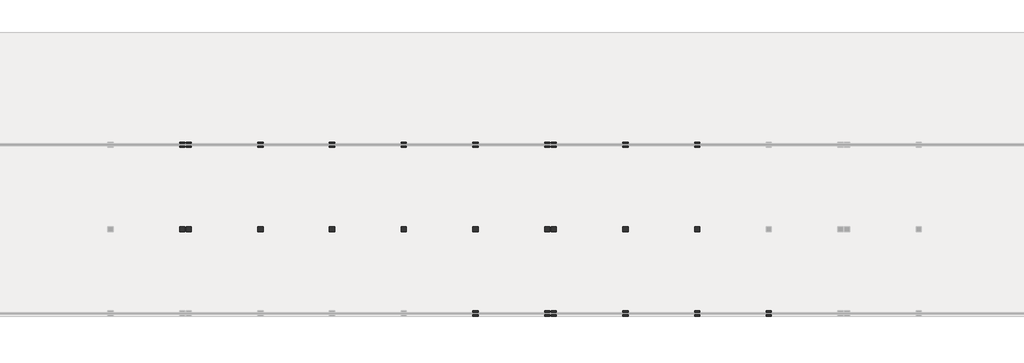
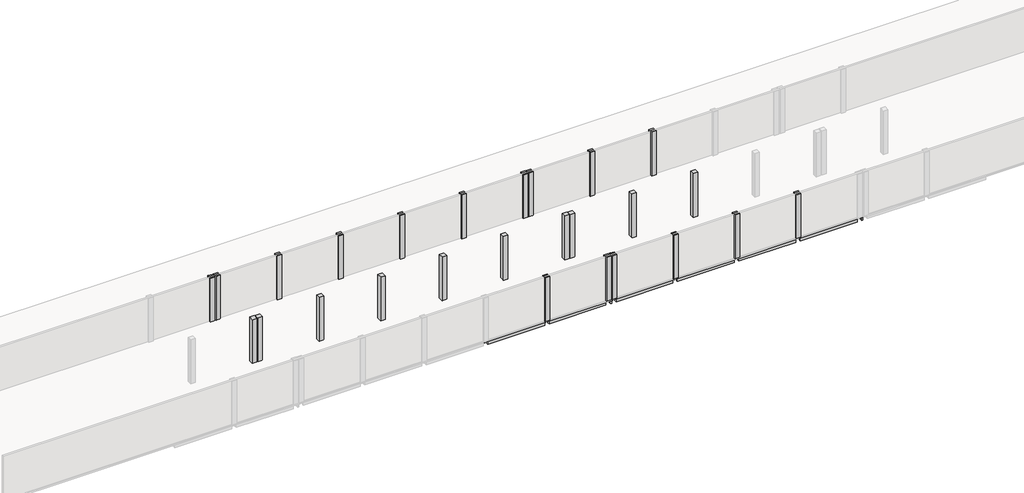
# One storey, part 2 of 4: 52 beams, 26 columns.
"""IFC4 building model written with IfcOpenShell, lengths in millimetres."""

from ifc_helpers import new_model, si_unit, frame, origin, place, context, project, spatial, polyline, outline, extrude, element, save

model = new_model("IFC4")

# Units and contexts
model_context = context("Model", 3, world=origin())
ifc_project = project(units=[si_unit("LENGTHUNIT", "METRE", prefix="MILLI")], contexts=[model_context])

# Site, building, storey
site = spatial("IfcSite", under=ifc_project)
building = spatial("IfcBuilding", under=site)
storey = spatial("IfcBuildingStorey", under=building, Name="03_T.O.C_1", Elevation=6949.9618634)

# Beams
placement = place(None, origin())
element("IfcBeam", 1, ObjectType="RC Beam_Rectangular : H_SB_AR_S16_B300xH600", at=placement, inside=storey, context=model_context, shape_type="SweptSolid", body=[
    extrude(outline(polyline([(35030.0, -6150.4791411), (35030.0, -5850.4791411), (35180.0, -5850.4791411), (35180.0, -6150.4791411), (35030.0, -6150.4791411)])), frame((0.0, 0.0, 6349.9618634), z_axis=(0.0, 0.0, 1.0), x_axis=(1.0, 0.0, 0.0)), (0.0, 0.0, 1.0), 499.0),
])
element("IfcBeam", 2, ObjectType="RC Beam_Rectangular : H_SB_AR_S16_B300xH600", at=placement, inside=storey, context=model_context, shape_type="SweptSolid", body=[
    extrude(outline(polyline([(35780.0, -6150.4791411), (35780.0, -5850.4791411), (43380.0, -5850.4791411), (43380.0, -6150.4791411), (35780.0, -6150.4791411)])), frame((0.0, 0.0, 6349.9618634), z_axis=(0.0, 0.0, 1.0), x_axis=(1.0, 0.0, 0.0)), (0.0, 0.0, 1.0), 499.0),
])
element("IfcBeam", 3, ObjectType="RC Beam_Rectangular : H_SB_AR_S16_B300xH600", at=placement, inside=storey, context=model_context, shape_type="SweptSolid", body=[
    extrude(outline(polyline([(43980.0, -6150.4791411), (43980.0, -5850.4791411), (51580.0, -5850.4791411), (51580.0, -6150.4791411), (43980.0, -6150.4791411)])), frame((0.0, 0.0, 6349.9618634), z_axis=(0.0, 0.0, 1.0), x_axis=(1.0, 0.0, 0.0)), (0.0, 0.0, 1.0), 499.0),
])
element("IfcBeam", 4, ObjectType="RC Beam_Rectangular : H_SB_AR_S16_B300xH600", at=placement, inside=storey, context=model_context, shape_type="SweptSolid", body=[
    extrude(outline(polyline([(52180.0, -6150.4791411), (52180.0, -5850.4791411), (59780.0, -5850.4791411), (59780.0, -6150.4791411), (52180.0, -6150.4791411)])), frame((0.0, 0.0, 6349.9618634), z_axis=(0.0, 0.0, 1.0), x_axis=(1.0, 0.0, 0.0)), (0.0, 0.0, 1.0), 499.0),
])
element("IfcBeam", 5, ObjectType="RC Beam_Rectangular : H_SB_AR_S16_B300xH600", at=placement, inside=storey, context=model_context, shape_type="SweptSolid", body=[
    extrude(outline(polyline([(60380.0, -6150.4791411), (60380.0, -5850.4791411), (67980.0, -5850.4791411), (67980.0, -6150.4791411), (60380.0, -6150.4791411)])), frame((0.0, 0.0, 6349.9618634), z_axis=(0.0, 0.0, 1.0), x_axis=(1.0, 0.0, 0.0)), (0.0, 0.0, 1.0), 499.0),
])
element("IfcBeam", 6, ObjectType="RC Beam_Rectangular : H_SB_AR_S16_B300xH600", at=placement, inside=storey, context=model_context, shape_type="SweptSolid", body=[
    extrude(outline(polyline([(68580.0, -6150.4791411), (68580.0, -5850.4791411), (76180.0, -5850.4791411), (76180.0, -6150.4791411), (68580.0, -6150.4791411)])), frame((0.0, 0.0, 6349.9618634), z_axis=(0.0, 0.0, 1.0), x_axis=(1.0, 0.0, 0.0)), (0.0, 0.0, 1.0), 499.0),
])
element("IfcBeam", 7, ObjectType="RC Beam_Rectangular : H_SB_AR_S16_B300xH600", at=placement, inside=storey, context=model_context, shape_type="SweptSolid", body=[
    extrude(outline(polyline([(76780.0, -6150.4791411), (76780.0, -5850.4791411), (76930.0, -5850.4791411), (76930.0, -6150.4791411), (76780.0, -6150.4791411)])), frame((0.0, 0.0, 6349.9618634), z_axis=(0.0, 0.0, 1.0), x_axis=(1.0, 0.0, 0.0)), (0.0, 0.0, 1.0), 499.0),
])
element("IfcBeam", 8, ObjectType="RC Beam_Rectangular : H_SB_AR_S16_B300xH600", at=placement, inside=storey, context=model_context, shape_type="SweptSolid", body=[
    extrude(outline(polyline([(77530.0, -6150.4791411), (77530.0, -5850.4791411), (85130.0, -5850.4791411), (85130.0, -6150.4791411), (77530.0, -6150.4791411)])), frame((0.0, 0.0, 6349.9618634), z_axis=(0.0, 0.0, 1.0), x_axis=(1.0, 0.0, 0.0)), (0.0, 0.0, 1.0), 499.0),
])
element("IfcBeam", 9, ObjectType="RC Beam_Rectangular : H_SB_AR_S16_B300xH600", at=placement, inside=storey, context=model_context, shape_type="SweptSolid", body=[
    extrude(outline(polyline([(85730.0, -6150.4791411), (85730.0, -5850.4791411), (93330.0, -5850.4791411), (93330.0, -6150.4791411), (85730.0, -6150.4791411)])), frame((0.0, 0.0, 6349.9618634), z_axis=(0.0, 0.0, 1.0), x_axis=(1.0, 0.0, 0.0)), (0.0, 0.0, 1.0), 499.0),
])
element("IfcBeam", 10, ObjectType="RC Beam_Rectangular : H_SB_AR_S16_B300xH600", at=placement, inside=storey, context=model_context, shape_type="SweptSolid", body=[
    extrude(outline(polyline([(35030.0, -15800.4791411), (35030.0, -15500.4791411), (35180.0, -15500.4791411), (35180.0, -15800.4791411), (35030.0, -15800.4791411)])), frame((0.0, 0.0, 6349.9618634), z_axis=(0.0, 0.0, 1.0), x_axis=(1.0, 0.0, 0.0)), (0.0, 0.0, 1.0), 499.0),
])
element("IfcBeam", 11, ObjectType="RC Beam_Rectangular : H_SB_AR_S16_B300xH600", at=placement, inside=storey, context=model_context, shape_type="SweptSolid", body=[
    extrude(outline(polyline([(35780.0, -15800.4791411), (35780.0, -15500.4791411), (43380.0, -15500.4791411), (43380.0, -15800.4791411), (35780.0, -15800.4791411)])), frame((0.0, 0.0, 6349.9618634), z_axis=(0.0, 0.0, 1.0), x_axis=(1.0, 0.0, 0.0)), (0.0, 0.0, 1.0), 499.0),
])
element("IfcBeam", 12, ObjectType="RC Beam_Rectangular : H_SB_AR_S16_B300xH600", at=placement, inside=storey, context=model_context, shape_type="SweptSolid", body=[
    extrude(outline(polyline([(43980.0, -15800.4791411), (43980.0, -15500.4791411), (51580.0, -15500.4791411), (51580.0, -15800.4791411), (43980.0, -15800.4791411)])), frame((0.0, 0.0, 6349.9618634), z_axis=(0.0, 0.0, 1.0), x_axis=(1.0, 0.0, 0.0)), (0.0, 0.0, 1.0), 499.0),
])
element("IfcBeam", 13, ObjectType="RC Beam_Rectangular : H_SB_AR_S16_B300xH600", at=placement, inside=storey, context=model_context, shape_type="SweptSolid", body=[
    extrude(outline(polyline([(52180.0, -15800.4791411), (52180.0, -15500.4791411), (59780.0, -15500.4791411), (59780.0, -15800.4791411), (52180.0, -15800.4791411)])), frame((0.0, 0.0, 6349.9618634), z_axis=(0.0, 0.0, 1.0), x_axis=(1.0, 0.0, 0.0)), (0.0, 0.0, 1.0), 499.0),
])
element("IfcBeam", 14, ObjectType="RC Beam_Rectangular : H_SB_AR_S16_B300xH600", at=placement, inside=storey, context=model_context, shape_type="SweptSolid", body=[
    extrude(outline(polyline([(60380.0, -15800.4791411), (60380.0, -15500.4791411), (67980.0, -15500.4791411), (67980.0, -15800.4791411), (60380.0, -15800.4791411)])), frame((0.0, 0.0, 6349.9618634), z_axis=(0.0, 0.0, 1.0), x_axis=(1.0, 0.0, 0.0)), (0.0, 0.0, 1.0), 499.0),
])
element("IfcBeam", 15, ObjectType="RC Beam_Rectangular : H_SB_AR_S16_B300xH600", at=placement, inside=storey, context=model_context, shape_type="SweptSolid", body=[
    extrude(outline(polyline([(68580.0, -15800.4791411), (68580.0, -15500.4791411), (76180.0, -15500.4791411), (76180.0, -15800.4791411), (68580.0, -15800.4791411)])), frame((0.0, 0.0, 6349.9618634), z_axis=(0.0, 0.0, 1.0), x_axis=(1.0, 0.0, 0.0)), (0.0, 0.0, 1.0), 499.0),
])
element("IfcBeam", 16, ObjectType="RC Beam_Rectangular : H_SB_AR_S16_B300xH600", at=placement, inside=storey, context=model_context, shape_type="SweptSolid", body=[
    extrude(outline(polyline([(76780.0, -15800.4791411), (76780.0, -15500.4791411), (76930.0, -15500.4791411), (76930.0, -15800.4791411), (76780.0, -15800.4791411)])), frame((0.0, 0.0, 6349.9618634), z_axis=(0.0, 0.0, 1.0), x_axis=(1.0, 0.0, 0.0)), (0.0, 0.0, 1.0), 499.0),
])
element("IfcBeam", 17, ObjectType="RC Beam_Rectangular : H_SB_AR_S16_B300xH600", at=placement, inside=storey, context=model_context, shape_type="SweptSolid", body=[
    extrude(outline(polyline([(77530.0, -15800.4791411), (77530.0, -15500.4791411), (85130.0, -15500.4791411), (85130.0, -15800.4791411), (77530.0, -15800.4791411)])), frame((0.0, 0.0, 6349.9618634), z_axis=(0.0, 0.0, 1.0), x_axis=(1.0, 0.0, 0.0)), (0.0, 0.0, 1.0), 499.0),
])
element("IfcBeam", 18, ObjectType="RC Beam_Rectangular : H_SB_AR_S16_B300xH600", at=placement, inside=storey, context=model_context, shape_type="SweptSolid", body=[
    extrude(outline(polyline([(85730.0, -15800.4791411), (85730.0, -15500.4791411), (93330.0, -15500.4791411), (93330.0, -15800.4791411), (85730.0, -15800.4791411)])), frame((0.0, 0.0, 6349.9618634), z_axis=(0.0, 0.0, 1.0), x_axis=(1.0, 0.0, 0.0)), (0.0, 0.0, 1.0), 499.0),
])
element("IfcBeam", 19, ObjectType="RC Beam_Rectangular : H_SB_AR_S16_B300xH600", at=placement, inside=storey, context=model_context, shape_type="SweptSolid", body=[
    extrude(outline(polyline([(60380.0, -25450.4791411), (60380.0, -25150.4791411), (67980.0, -25150.4791411), (67980.0, -25450.4791411), (60380.0, -25450.4791411)])), frame((0.0, 0.0, 6349.9618634), z_axis=(0.0, 0.0, 1.0), x_axis=(1.0, 0.0, 0.0)), (0.0, 0.0, 1.0), 499.0),
])
element("IfcBeam", 20, ObjectType="RC Beam_Rectangular : H_SB_AR_S16_B300xH600", at=placement, inside=storey, context=model_context, shape_type="SweptSolid", body=[
    extrude(outline(polyline([(68580.0, -25450.4791411), (68580.0, -25150.4791411), (76180.0, -25150.4791411), (76180.0, -25450.4791411), (68580.0, -25450.4791411)])), frame((0.0, 0.0, 6349.9618634), z_axis=(0.0, 0.0, 1.0), x_axis=(1.0, 0.0, 0.0)), (0.0, 0.0, 1.0), 499.0),
])
element("IfcBeam", 21, ObjectType="RC Beam_Rectangular : H_SB_AR_S16_B300xH600", at=placement, inside=storey, context=model_context, shape_type="SweptSolid", body=[
    extrude(outline(polyline([(76780.0, -25450.4791411), (76780.0, -25150.4791411), (76930.0, -25150.4791411), (76930.0, -25450.4791411), (76780.0, -25450.4791411)])), frame((0.0, 0.0, 6349.9618634), z_axis=(0.0, 0.0, 1.0), x_axis=(1.0, 0.0, 0.0)), (0.0, 0.0, 1.0), 499.0),
])
element("IfcBeam", 22, ObjectType="RC Beam_Rectangular : H_SB_AR_S16_B300xH600", at=placement, inside=storey, context=model_context, shape_type="SweptSolid", body=[
    extrude(outline(polyline([(77530.0, -25450.4791411), (77530.0, -25150.4791411), (85130.0, -25150.4791411), (85130.0, -25450.4791411), (77530.0, -25450.4791411)])), frame((0.0, 0.0, 6349.9618634), z_axis=(0.0, 0.0, 1.0), x_axis=(1.0, 0.0, 0.0)), (0.0, 0.0, 1.0), 499.0),
])
element("IfcBeam", 23, ObjectType="RC Beam_Rectangular : H_SB_AR_S16_B300xH600", at=placement, inside=storey, context=model_context, shape_type="SweptSolid", body=[
    extrude(outline(polyline([(85730.0, -25450.4791411), (85730.0, -25150.4791411), (93330.0, -25150.4791411), (93330.0, -25450.4791411), (85730.0, -25450.4791411)])), frame((0.0, 0.0, 6349.9618634), z_axis=(0.0, 0.0, 1.0), x_axis=(1.0, 0.0, 0.0)), (0.0, 0.0, 1.0), 499.0),
])
element("IfcBeam", 24, ObjectType="RC Beam_Rectangular : H_SB_AR_S16_B300xH600", at=placement, inside=storey, context=model_context, shape_type="SweptSolid", body=[
    extrude(outline(polyline([(93930.0, -25450.4791411), (93930.0, -25150.4791411), (101530.0, -25150.4791411), (101530.0, -25450.4791411), (93930.0, -25450.4791411)])), frame((0.0, 0.0, 6349.9618634), z_axis=(0.0, 0.0, 1.0), x_axis=(1.0, 0.0, 0.0)), (0.0, 0.0, 1.0), 499.0),
])
element("IfcBeam", 25, ObjectType="RC Beam_Rectangular : H_SB_AR_S16_B300xH600", at=placement, inside=storey, context=model_context, shape_type="SweptSolid", body=[
    extrude(outline(polyline([(102130.0, -25450.4791411), (102130.0, -25150.4791411), (109730.0, -25150.4791411), (109730.0, -25450.4791411), (102130.0, -25450.4791411)])), frame((0.0, 0.0, 6349.9618634), z_axis=(0.0, 0.0, 1.0), x_axis=(1.0, 0.0, 0.0)), (0.0, 0.0, 1.0), 499.0),
])
element("IfcBeam", 26, ObjectType="RC Beam_Rectangular : H_SB_AR_S16_B300xH600", at=placement, inside=storey, context=model_context, shape_type="SweptSolid", body=[
    extrude(outline(polyline([(110330.0, -25450.4791411), (110330.0, -25150.4791411), (110480.0, -25150.4791411), (110480.0, -25450.4791411), (110330.0, -25450.4791411)])), frame((0.0, 0.0, 6349.9618634), z_axis=(0.0, 0.0, 1.0), x_axis=(1.0, 0.0, 0.0)), (0.0, 0.0, 1.0), 499.0),
])
element("IfcBeam", 27, ObjectType="RC Beam_Rectangular : H_SB_AR_S16_B300xH600", at=placement, inside=storey, context=model_context, shape_type="SweptSolid", body=[
    extrude(outline(polyline([(34580.0, -6300.4791411), (34880.0, -6300.4791411), (34880.0, -15350.4791411), (34580.0, -15350.4791411), (34580.0, -6300.4791411)])), frame((0.0, 0.0, 6349.9618634), z_axis=(0.0, 0.0, 1.0), x_axis=(1.0, 0.0, 0.0)), (0.0, 0.0, 1.0), 499.0),
])
element("IfcBeam", 28, ObjectType="RC Beam_Rectangular : H_SB_AR_S16_B300xH600", at=placement, inside=storey, context=model_context, shape_type="SweptSolid", body=[
    extrude(outline(polyline([(34580.0, -50.4791411), (34880.0, -50.4791411), (34880.0, -5700.4791411), (34580.0, -5700.4791411), (34580.0, -50.4791411)])), frame((0.0, 0.0, 6349.9618634), z_axis=(0.0, 0.0, 1.0), x_axis=(1.0, 0.0, 0.0)), (0.0, 0.0, 1.0), 499.0),
])
element("IfcBeam", 29, ObjectType="RC Beam_Rectangular : H_SB_AR_S16_B300xH600", at=placement, inside=storey, context=model_context, shape_type="SweptSolid", body=[
    extrude(outline(polyline([(35330.0, -6300.4791411), (35630.0, -6300.4791411), (35630.0, -15350.4791411), (35330.0, -15350.4791411), (35330.0, -6300.4791411)])), frame((0.0, 0.0, 6349.9618634), z_axis=(0.0, 0.0, 1.0), x_axis=(1.0, 0.0, 0.0)), (0.0, 0.0, 1.0), 499.0),
])
element("IfcBeam", 30, ObjectType="RC Beam_Rectangular : H_SB_AR_S16_B300xH600", at=placement, inside=storey, context=model_context, shape_type="SweptSolid", body=[
    extrude(outline(polyline([(35330.0, 99.5208589), (35630.0, 99.5208589), (35630.0, -5700.4791411), (35330.0, -5700.4791411), (35330.0, 99.5208589)])), frame((0.0, 0.0, 6349.9618634), z_axis=(0.0, 0.0, 1.0), x_axis=(1.0, 0.0, 0.0)), (0.0, 0.0, 1.0), 499.0),
])
element("IfcBeam", 31, ObjectType="RC Beam_Rectangular : H_SB_AR_S16_B300xH600", at=placement, inside=storey, context=model_context, shape_type="SweptSolid", body=[
    extrude(outline(polyline([(43530.0, -6300.4791411), (43830.0, -6300.4791411), (43830.0, -15350.4791411), (43530.0, -15350.4791411), (43530.0, -6300.4791411)])), frame((0.0, 0.0, 6349.9618634), z_axis=(0.0, 0.0, 1.0), x_axis=(1.0, 0.0, 0.0)), (0.0, 0.0, 1.0), 499.0),
])
element("IfcBeam", 32, ObjectType="RC Beam_Rectangular : H_SB_AR_S16_B300xH600", at=placement, inside=storey, context=model_context, shape_type="SweptSolid", body=[
    extrude(outline(polyline([(43530.0, 99.5208589), (43830.0, 99.5208589), (43830.0, -5700.4791411), (43530.0, -5700.4791411), (43530.0, 99.5208589)])), frame((0.0, 0.0, 6349.9618634), z_axis=(0.0, 0.0, 1.0), x_axis=(1.0, 0.0, 0.0)), (0.0, 0.0, 1.0), 499.0),
])
element("IfcBeam", 33, ObjectType="RC Beam_Rectangular : H_SB_AR_S16_B300xH600", at=placement, inside=storey, context=model_context, shape_type="SweptSolid", body=[
    extrude(outline(polyline([(51730.0, -6300.4791411), (52030.0, -6300.4791411), (52030.0, -15350.4791411), (51730.0, -15350.4791411), (51730.0, -6300.4791411)])), frame((0.0, 0.0, 6349.9618634), z_axis=(0.0, 0.0, 1.0), x_axis=(1.0, 0.0, 0.0)), (0.0, 0.0, 1.0), 499.0),
])
element("IfcBeam", 34, ObjectType="RC Beam_Rectangular : H_SB_AR_S16_B300xH600", at=placement, inside=storey, context=model_context, shape_type="SweptSolid", body=[
    extrude(outline(polyline([(51730.0, 99.5208589), (52030.0, 99.5208589), (52030.0, -5700.4791411), (51730.0, -5700.4791411), (51730.0, 99.5208589)])), frame((0.0, 0.0, 6349.9618634), z_axis=(0.0, 0.0, 1.0), x_axis=(1.0, 0.0, 0.0)), (0.0, 0.0, 1.0), 499.0),
])
element("IfcBeam", 35, ObjectType="RC Beam_Rectangular : H_SB_AR_S16_B300xH600", at=placement, inside=storey, context=model_context, shape_type="SweptSolid", body=[
    extrude(outline(polyline([(59930.0, -15950.4791411), (60230.0, -15950.4791411), (60230.0, -25000.4791411), (59930.0, -25000.4791411), (59930.0, -15950.4791411)])), frame((0.0, 0.0, 6349.9618634), z_axis=(0.0, 0.0, 1.0), x_axis=(1.0, 0.0, 0.0)), (0.0, 0.0, 1.0), 499.0),
])
element("IfcBeam", 36, ObjectType="RC Beam_Rectangular : H_SB_AR_S16_B300xH600", at=placement, inside=storey, context=model_context, shape_type="SweptSolid", body=[
    extrude(outline(polyline([(59930.0, -6300.4791411), (60230.0, -6300.4791411), (60230.0, -15350.4791411), (59930.0, -15350.4791411), (59930.0, -6300.4791411)])), frame((0.0, 0.0, 6349.9618634), z_axis=(0.0, 0.0, 1.0), x_axis=(1.0, 0.0, 0.0)), (0.0, 0.0, 1.0), 499.0),
])
element("IfcBeam", 37, ObjectType="RC Beam_Rectangular : H_SB_AR_S16_B300xH600", at=placement, inside=storey, context=model_context, shape_type="SweptSolid", body=[
    extrude(outline(polyline([(59930.0, 99.5208589), (60230.0, 99.5208589), (60230.0, -5700.4791411), (59930.0, -5700.4791411), (59930.0, 99.5208589)])), frame((0.0, 0.0, 6349.9618634), z_axis=(0.0, 0.0, 1.0), x_axis=(1.0, 0.0, 0.0)), (0.0, 0.0, 1.0), 499.0),
])
element("IfcBeam", 38, ObjectType="RC Beam_Rectangular : H_SB_AR_S16_B300xH600", at=placement, inside=storey, context=model_context, shape_type="SweptSolid", body=[
    extrude(outline(polyline([(68130.0, -15950.4791411), (68430.0, -15950.4791411), (68430.0, -25000.4791411), (68130.0, -25000.4791411), (68130.0, -15950.4791411)])), frame((0.0, 0.0, 6349.9618634), z_axis=(0.0, 0.0, 1.0), x_axis=(1.0, 0.0, 0.0)), (0.0, 0.0, 1.0), 499.0),
])
element("IfcBeam", 39, ObjectType="RC Beam_Rectangular : H_SB_AR_S16_B300xH600", at=placement, inside=storey, context=model_context, shape_type="SweptSolid", body=[
    extrude(outline(polyline([(68130.0, -6300.4791411), (68430.0, -6300.4791411), (68430.0, -15350.4791411), (68130.0, -15350.4791411), (68130.0, -6300.4791411)])), frame((0.0, 0.0, 6349.9618634), z_axis=(0.0, 0.0, 1.0), x_axis=(1.0, 0.0, 0.0)), (0.0, 0.0, 1.0), 499.0),
])
element("IfcBeam", 40, ObjectType="RC Beam_Rectangular : H_SB_AR_S16_B300xH600", at=placement, inside=storey, context=model_context, shape_type="SweptSolid", body=[
    extrude(outline(polyline([(68130.0, 99.5208589), (68430.0, 99.5208589), (68430.0, -5700.4791411), (68130.0, -5700.4791411), (68130.0, 99.5208589)])), frame((0.0, 0.0, 6349.9618634), z_axis=(0.0, 0.0, 1.0), x_axis=(1.0, 0.0, 0.0)), (0.0, 0.0, 1.0), 499.0),
])
element("IfcBeam", 41, ObjectType="RC Beam_Rectangular : H_SB_AR_S16_B300xH600", at=placement, inside=storey, context=model_context, shape_type="SweptSolid", body=[
    extrude(outline(polyline([(76330.0, -15950.4791411), (76630.0, -15950.4791411), (76630.0, -25000.4791411), (76330.0, -25000.4791411), (76330.0, -15950.4791411)])), frame((0.0, 0.0, 6349.9618634), z_axis=(0.0, 0.0, 1.0), x_axis=(1.0, 0.0, 0.0)), (0.0, 0.0, 1.0), 499.0),
])
element("IfcBeam", 42, ObjectType="RC Beam_Rectangular : H_SB_AR_S16_B300xH600", at=placement, inside=storey, context=model_context, shape_type="SweptSolid", body=[
    extrude(outline(polyline([(76330.0, -6300.4791411), (76630.0, -6300.4791411), (76630.0, -15350.4791411), (76330.0, -15350.4791411), (76330.0, -6300.4791411)])), frame((0.0, 0.0, 6349.9618634), z_axis=(0.0, 0.0, 1.0), x_axis=(1.0, 0.0, 0.0)), (0.0, 0.0, 1.0), 499.0),
])
element("IfcBeam", 43, ObjectType="RC Beam_Rectangular : H_SB_AR_S16_B300xH600", at=placement, inside=storey, context=model_context, shape_type="SweptSolid", body=[
    extrude(outline(polyline([(76330.0, 99.5208589), (76630.0, 99.5208589), (76630.0, -5700.4791411), (76330.0, -5700.4791411), (76330.0, 99.5208589)])), frame((0.0, 0.0, 6349.9618634), z_axis=(0.0, 0.0, 1.0), x_axis=(1.0, 0.0, 0.0)), (0.0, 0.0, 1.0), 499.0),
])
element("IfcBeam", 44, ObjectType="RC Beam_Rectangular : H_SB_AR_S16_B300xH600", at=placement, inside=storey, context=model_context, shape_type="SweptSolid", body=[
    extrude(outline(polyline([(77080.0, -15950.4791411), (77380.0, -15950.4791411), (77380.0, -25000.4791411), (77080.0, -25000.4791411), (77080.0, -15950.4791411)])), frame((0.0, 0.0, 6349.9618634), z_axis=(0.0, 0.0, 1.0), x_axis=(1.0, 0.0, 0.0)), (0.0, 0.0, 1.0), 499.0),
])
element("IfcBeam", 45, ObjectType="RC Beam_Rectangular : H_SB_AR_S16_B300xH600", at=placement, inside=storey, context=model_context, shape_type="SweptSolid", body=[
    extrude(outline(polyline([(77080.0, -6300.4791411), (77380.0, -6300.4791411), (77380.0, -15350.4791411), (77080.0, -15350.4791411), (77080.0, -6300.4791411)])), frame((0.0, 0.0, 6349.9618634), z_axis=(0.0, 0.0, 1.0), x_axis=(1.0, 0.0, 0.0)), (0.0, 0.0, 1.0), 499.0),
])
element("IfcBeam", 46, ObjectType="RC Beam_Rectangular : H_SB_AR_S16_B300xH600", at=placement, inside=storey, context=model_context, shape_type="SweptSolid", body=[
    extrude(outline(polyline([(77080.0, 99.5208589), (77380.0, 99.5208589), (77380.0, -5700.4791411), (77080.0, -5700.4791411), (77080.0, 99.5208589)])), frame((0.0, 0.0, 6349.9618634), z_axis=(0.0, 0.0, 1.0), x_axis=(1.0, 0.0, 0.0)), (0.0, 0.0, 1.0), 499.0),
])
element("IfcBeam", 47, ObjectType="RC Beam_Rectangular : H_SB_AR_S16_B300xH600", at=placement, inside=storey, context=model_context, shape_type="SweptSolid", body=[
    extrude(outline(polyline([(85280.0, -15950.4791411), (85580.0, -15950.4791411), (85580.0, -25000.4791411), (85280.0, -25000.4791411), (85280.0, -15950.4791411)])), frame((0.0, 0.0, 6349.9618634), z_axis=(0.0, 0.0, 1.0), x_axis=(1.0, 0.0, 0.0)), (0.0, 0.0, 1.0), 499.0),
])
element("IfcBeam", 48, ObjectType="RC Beam_Rectangular : H_SB_AR_S16_B300xH600", at=placement, inside=storey, context=model_context, shape_type="SweptSolid", body=[
    extrude(outline(polyline([(85280.0, -6300.4791411), (85580.0, -6300.4791411), (85580.0, -15350.4791411), (85280.0, -15350.4791411), (85280.0, -6300.4791411)])), frame((0.0, 0.0, 6349.9618634), z_axis=(0.0, 0.0, 1.0), x_axis=(1.0, 0.0, 0.0)), (0.0, 0.0, 1.0), 499.0),
])
element("IfcBeam", 49, ObjectType="RC Beam_Rectangular : H_SB_AR_S16_B300xH600", at=placement, inside=storey, context=model_context, shape_type="SweptSolid", body=[
    extrude(outline(polyline([(85280.0, 99.5208589), (85580.0, 99.5208589), (85580.0, -5700.4791411), (85280.0, -5700.4791411), (85280.0, 99.5208589)])), frame((0.0, 0.0, 6349.9618634), z_axis=(0.0, 0.0, 1.0), x_axis=(1.0, 0.0, 0.0)), (0.0, 0.0, 1.0), 499.0),
])
element("IfcBeam", 50, ObjectType="RC Beam_Rectangular : H_SB_AR_S16_B300xH600", at=placement, inside=storey, context=model_context, shape_type="SweptSolid", body=[
    extrude(outline(polyline([(93480.0, -15950.4791411), (93780.0, -15950.4791411), (93780.0, -25000.4791411), (93480.0, -25000.4791411), (93480.0, -15950.4791411)])), frame((0.0, 0.0, 6349.9618634), z_axis=(0.0, 0.0, 1.0), x_axis=(1.0, 0.0, 0.0)), (0.0, 0.0, 1.0), 499.0),
])
element("IfcBeam", 51, ObjectType="RC Beam_Rectangular : H_SB_AR_S16_B300xH600", at=placement, inside=storey, context=model_context, shape_type="SweptSolid", body=[
    extrude(outline(polyline([(93480.0, -6300.4791411), (93780.0, -6300.4791411), (93780.0, -15350.4791411), (93480.0, -15350.4791411), (93480.0, -6300.4791411)])), frame((0.0, 0.0, 6349.9618634), z_axis=(0.0, 0.0, 1.0), x_axis=(1.0, 0.0, 0.0)), (0.0, 0.0, 1.0), 499.0),
])
element("IfcBeam", 52, ObjectType="RC Beam_Rectangular : H_SB_AR_S16_B300xH600", at=placement, inside=storey, context=model_context, shape_type="SweptSolid", body=[
    extrude(outline(polyline([(93480.0, 99.5208589), (93780.0, 99.5208589), (93780.0, -5700.4791411), (93480.0, -5700.4791411), (93480.0, 99.5208589)])), frame((0.0, 0.0, 6349.9618634), z_axis=(0.0, 0.0, 1.0), x_axis=(1.0, 0.0, 0.0)), (0.0, 0.0, 1.0), 499.0),
])

# Columns
element("IfcColumn", 53, ObjectType="RC_Column_Rectangular : H_SC_AR_S15_W600xL600", at=placement, inside=storey, context=model_context, shape_type="SweptSolid", body=[
    extrude(outline(polyline([(35030.0, -5700.4791411), (35030.0, -6300.4791411), (34430.0, -6300.4791411), (34430.0, -5700.4791411), (35030.0, -5700.4791411)])), frame((0.0, 0.0, 6949.9618634), z_axis=(0.0, 0.0, 1.0), x_axis=(1.0, 0.0, 0.0)), (0.0, 0.0, 1.0), 6200.0),
])
element("IfcColumn", 54, ObjectType="RC_Column_Rectangular : H_SC_AR_S15_W600xL600", at=placement, inside=storey, context=model_context, shape_type="SweptSolid", body=[
    extrude(outline(polyline([(35780.0, -5700.4791411), (35780.0, -6300.4791411), (35180.0, -6300.4791411), (35180.0, -5700.4791411), (35780.0, -5700.4791411)])), frame((0.0, 0.0, 6949.9618634), z_axis=(0.0, 0.0, 1.0), x_axis=(1.0, 0.0, 0.0)), (0.0, 0.0, 1.0), 6200.0),
])
element("IfcColumn", 55, ObjectType="RC_Column_Rectangular : H_SC_AR_S15_W600xL600", at=placement, inside=storey, context=model_context, shape_type="SweptSolid", body=[
    extrude(outline(polyline([(43980.0, -5700.4791411), (43980.0, -6300.4791411), (43380.0, -6300.4791411), (43380.0, -5700.4791411), (43980.0, -5700.4791411)])), frame((0.0, 0.0, 6949.9618634), z_axis=(0.0, 0.0, 1.0), x_axis=(1.0, 0.0, 0.0)), (0.0, 0.0, 1.0), 6200.0),
])
element("IfcColumn", 56, ObjectType="RC_Column_Rectangular : H_SC_AR_S15_W600xL600", at=placement, inside=storey, context=model_context, shape_type="SweptSolid", body=[
    extrude(outline(polyline([(52180.0, -5700.4791411), (52180.0, -6300.4791411), (51580.0, -6300.4791411), (51580.0, -5700.4791411), (52180.0, -5700.4791411)])), frame((0.0, 0.0, 6949.9618634), z_axis=(0.0, 0.0, 1.0), x_axis=(1.0, 0.0, 0.0)), (0.0, 0.0, 1.0), 6200.0),
])
element("IfcColumn", 57, ObjectType="RC_Column_Rectangular : H_SC_AR_S15_W600xL600", at=placement, inside=storey, context=model_context, shape_type="SweptSolid", body=[
    extrude(outline(polyline([(60380.0, -5700.4791411), (60380.0, -6300.4791411), (59780.0, -6300.4791411), (59780.0, -5700.4791411), (60380.0, -5700.4791411)])), frame((0.0, 0.0, 6949.9618634), z_axis=(0.0, 0.0, 1.0), x_axis=(1.0, 0.0, 0.0)), (0.0, 0.0, 1.0), 6200.0),
])
element("IfcColumn", 58, ObjectType="RC_Column_Rectangular : H_SC_AR_S15_W600xL600", at=placement, inside=storey, context=model_context, shape_type="SweptSolid", body=[
    extrude(outline(polyline([(68580.0, -5700.4791411), (68580.0, -6300.4791411), (67980.0, -6300.4791411), (67980.0, -5700.4791411), (68580.0, -5700.4791411)])), frame((0.0, 0.0, 6949.9618634), z_axis=(0.0, 0.0, 1.0), x_axis=(1.0, 0.0, 0.0)), (0.0, 0.0, 1.0), 6200.0),
])
element("IfcColumn", 59, ObjectType="RC_Column_Rectangular : H_SC_AR_S15_W600xL600", at=placement, inside=storey, context=model_context, shape_type="SweptSolid", body=[
    extrude(outline(polyline([(76780.0, -5700.4791411), (76780.0, -6300.4791411), (76180.0, -6300.4791411), (76180.0, -5700.4791411), (76780.0, -5700.4791411)])), frame((0.0, 0.0, 6949.9618634), z_axis=(0.0, 0.0, 1.0), x_axis=(1.0, 0.0, 0.0)), (0.0, 0.0, 1.0), 6200.0),
])
element("IfcColumn", 60, ObjectType="RC_Column_Rectangular : H_SC_AR_S15_W600xL600", at=placement, inside=storey, context=model_context, shape_type="SweptSolid", body=[
    extrude(outline(polyline([(77530.0, -5700.4791411), (77530.0, -6300.4791411), (76930.0, -6300.4791411), (76930.0, -5700.4791411), (77530.0, -5700.4791411)])), frame((0.0, 0.0, 6949.9618634), z_axis=(0.0, 0.0, 1.0), x_axis=(1.0, 0.0, 0.0)), (0.0, 0.0, 1.0), 6200.0),
])
element("IfcColumn", 61, ObjectType="RC_Column_Rectangular : H_SC_AR_S15_W600xL600", at=placement, inside=storey, context=model_context, shape_type="SweptSolid", body=[
    extrude(outline(polyline([(85730.0, -5700.4791411), (85730.0, -6300.4791411), (85130.0, -6300.4791411), (85130.0, -5700.4791411), (85730.0, -5700.4791411)])), frame((0.0, 0.0, 6949.9618634), z_axis=(0.0, 0.0, 1.0), x_axis=(1.0, 0.0, 0.0)), (0.0, 0.0, 1.0), 6200.0),
])
element("IfcColumn", 62, ObjectType="RC_Column_Rectangular : H_SC_AR_S15_W600xL600", at=placement, inside=storey, context=model_context, shape_type="SweptSolid", body=[
    extrude(outline(polyline([(93930.0, -5700.4791411), (93930.0, -6300.4791411), (93330.0, -6300.4791411), (93330.0, -5700.4791411), (93930.0, -5700.4791411)])), frame((0.0, 0.0, 6949.9618634), z_axis=(0.0, 0.0, 1.0), x_axis=(1.0, 0.0, 0.0)), (0.0, 0.0, 1.0), 6200.0),
])
element("IfcColumn", 63, ObjectType="RC_Column_Rectangular : H_SC_AR_S15_W600xL600", at=placement, inside=storey, context=model_context, shape_type="SweptSolid", body=[
    extrude(outline(polyline([(35030.0, -15350.4791411), (35030.0, -15950.4791411), (34430.0, -15950.4791411), (34430.0, -15350.4791411), (35030.0, -15350.4791411)])), frame((0.0, 0.0, 6949.9618634), z_axis=(0.0, 0.0, 1.0), x_axis=(1.0, 0.0, 0.0)), (0.0, 0.0, 1.0), 6200.0),
])
element("IfcColumn", 64, ObjectType="RC_Column_Rectangular : H_SC_AR_S15_W600xL600", at=placement, inside=storey, context=model_context, shape_type="SweptSolid", body=[
    extrude(outline(polyline([(35780.0, -15350.4791411), (35780.0, -15950.4791411), (35180.0, -15950.4791411), (35180.0, -15350.4791411), (35780.0, -15350.4791411)])), frame((0.0, 0.0, 6949.9618634), z_axis=(0.0, 0.0, 1.0), x_axis=(1.0, 0.0, 0.0)), (0.0, 0.0, 1.0), 6200.0),
])
element("IfcColumn", 65, ObjectType="RC_Column_Rectangular : H_SC_AR_S15_W600xL600", at=placement, inside=storey, context=model_context, shape_type="SweptSolid", body=[
    extrude(outline(polyline([(43980.0, -15350.4791411), (43980.0, -15950.4791411), (43380.0, -15950.4791411), (43380.0, -15350.4791411), (43980.0, -15350.4791411)])), frame((0.0, 0.0, 6949.9618634), z_axis=(0.0, 0.0, 1.0), x_axis=(1.0, 0.0, 0.0)), (0.0, 0.0, 1.0), 6200.0),
])
element("IfcColumn", 66, ObjectType="RC_Column_Rectangular : H_SC_AR_S15_W600xL600", at=placement, inside=storey, context=model_context, shape_type="SweptSolid", body=[
    extrude(outline(polyline([(52180.0, -15350.4791411), (52180.0, -15950.4791411), (51580.0, -15950.4791411), (51580.0, -15350.4791411), (52180.0, -15350.4791411)])), frame((0.0, 0.0, 6949.9618634), z_axis=(0.0, 0.0, 1.0), x_axis=(1.0, 0.0, 0.0)), (0.0, 0.0, 1.0), 6200.0),
])
element("IfcColumn", 67, ObjectType="RC_Column_Rectangular : H_SC_AR_S15_W600xL600", at=placement, inside=storey, context=model_context, shape_type="SweptSolid", body=[
    extrude(outline(polyline([(60380.0, -15350.4791411), (60380.0, -15950.4791411), (59780.0, -15950.4791411), (59780.0, -15350.4791411), (60380.0, -15350.4791411)])), frame((0.0, 0.0, 6949.9618634), z_axis=(0.0, 0.0, 1.0), x_axis=(1.0, 0.0, 0.0)), (0.0, 0.0, 1.0), 6200.0),
])
element("IfcColumn", 68, ObjectType="RC_Column_Rectangular : H_SC_AR_S15_W600xL600", at=placement, inside=storey, context=model_context, shape_type="SweptSolid", body=[
    extrude(outline(polyline([(68580.0, -15350.4791411), (68580.0, -15950.4791411), (67980.0, -15950.4791411), (67980.0, -15350.4791411), (68580.0, -15350.4791411)])), frame((0.0, 0.0, 6949.9618634), z_axis=(0.0, 0.0, 1.0), x_axis=(1.0, 0.0, 0.0)), (0.0, 0.0, 1.0), 6200.0),
])
element("IfcColumn", 69, ObjectType="RC_Column_Rectangular : H_SC_AR_S15_W600xL600", at=placement, inside=storey, context=model_context, shape_type="SweptSolid", body=[
    extrude(outline(polyline([(76780.0, -15350.4791411), (76780.0, -15950.4791411), (76180.0, -15950.4791411), (76180.0, -15350.4791411), (76780.0, -15350.4791411)])), frame((0.0, 0.0, 6949.9618634), z_axis=(0.0, 0.0, 1.0), x_axis=(1.0, 0.0, 0.0)), (0.0, 0.0, 1.0), 6200.0),
])
element("IfcColumn", 70, ObjectType="RC_Column_Rectangular : H_SC_AR_S15_W600xL600", at=placement, inside=storey, context=model_context, shape_type="SweptSolid", body=[
    extrude(outline(polyline([(77530.0, -15350.4791411), (77530.0, -15950.4791411), (76930.0, -15950.4791411), (76930.0, -15350.4791411), (77530.0, -15350.4791411)])), frame((0.0, 0.0, 6949.9618634), z_axis=(0.0, 0.0, 1.0), x_axis=(1.0, 0.0, 0.0)), (0.0, 0.0, 1.0), 6200.0),
])
element("IfcColumn", 71, ObjectType="RC_Column_Rectangular : H_SC_AR_S15_W600xL600", at=placement, inside=storey, context=model_context, shape_type="SweptSolid", body=[
    extrude(outline(polyline([(85730.0, -15350.4791411), (85730.0, -15950.4791411), (85130.0, -15950.4791411), (85130.0, -15350.4791411), (85730.0, -15350.4791411)])), frame((0.0, 0.0, 6949.9618634), z_axis=(0.0, 0.0, 1.0), x_axis=(1.0, 0.0, 0.0)), (0.0, 0.0, 1.0), 6200.0),
])
element("IfcColumn", 72, ObjectType="RC_Column_Rectangular : H_SC_AR_S15_W600xL600", at=placement, inside=storey, context=model_context, shape_type="SweptSolid", body=[
    extrude(outline(polyline([(93930.0, -15350.4791411), (93930.0, -15950.4791411), (93330.0, -15950.4791411), (93330.0, -15350.4791411), (93930.0, -15350.4791411)])), frame((0.0, 0.0, 6949.9618634), z_axis=(0.0, 0.0, 1.0), x_axis=(1.0, 0.0, 0.0)), (0.0, 0.0, 1.0), 6200.0),
])
element("IfcColumn", 73, ObjectType="RC_Column_Rectangular : H_SC_AR_S15_W600xL600", at=placement, inside=storey, context=model_context, shape_type="SweptSolid", body=[
    extrude(outline(polyline([(68580.0, -25000.4791411), (68580.0, -25600.4791411), (67980.0, -25600.4791411), (67980.0, -25000.4791411), (68580.0, -25000.4791411)])), frame((0.0, 0.0, 6949.9618634), z_axis=(0.0, 0.0, 1.0), x_axis=(1.0, 0.0, 0.0)), (0.0, 0.0, 1.0), 6200.0),
])
element("IfcColumn", 74, ObjectType="RC_Column_Rectangular : H_SC_AR_S15_W600xL600", at=placement, inside=storey, context=model_context, shape_type="SweptSolid", body=[
    extrude(outline(polyline([(76780.0, -25000.4791411), (76780.0, -25600.4791411), (76180.0, -25600.4791411), (76180.0, -25000.4791411), (76780.0, -25000.4791411)])), frame((0.0, 0.0, 6949.9618634), z_axis=(0.0, 0.0, 1.0), x_axis=(1.0, 0.0, 0.0)), (0.0, 0.0, 1.0), 6200.0),
])
element("IfcColumn", 75, ObjectType="RC_Column_Rectangular : H_SC_AR_S15_W600xL600", at=placement, inside=storey, context=model_context, shape_type="SweptSolid", body=[
    extrude(outline(polyline([(77530.0, -25000.4791411), (77530.0, -25600.4791411), (76930.0, -25600.4791411), (76930.0, -25000.4791411), (77530.0, -25000.4791411)])), frame((0.0, 0.0, 6949.9618634), z_axis=(0.0, 0.0, 1.0), x_axis=(1.0, 0.0, 0.0)), (0.0, 0.0, 1.0), 6200.0),
])
element("IfcColumn", 76, ObjectType="RC_Column_Rectangular : H_SC_AR_S15_W600xL600", at=placement, inside=storey, context=model_context, shape_type="SweptSolid", body=[
    extrude(outline(polyline([(85730.0, -25000.4791411), (85730.0, -25600.4791411), (85130.0, -25600.4791411), (85130.0, -25000.4791411), (85730.0, -25000.4791411)])), frame((0.0, 0.0, 6949.9618634), z_axis=(0.0, 0.0, 1.0), x_axis=(1.0, 0.0, 0.0)), (0.0, 0.0, 1.0), 6200.0),
])
element("IfcColumn", 77, ObjectType="RC_Column_Rectangular : H_SC_AR_S15_W600xL600", at=placement, inside=storey, context=model_context, shape_type="SweptSolid", body=[
    extrude(outline(polyline([(93930.0, -25000.4791411), (93930.0, -25600.4791411), (93330.0, -25600.4791411), (93330.0, -25000.4791411), (93930.0, -25000.4791411)])), frame((0.0, 0.0, 6949.9618634), z_axis=(0.0, 0.0, 1.0), x_axis=(1.0, 0.0, 0.0)), (0.0, 0.0, 1.0), 6200.0),
])
element("IfcColumn", 78, ObjectType="RC_Column_Rectangular : H_SC_AR_S15_W600xL600", at=placement, inside=storey, context=model_context, shape_type="SweptSolid", body=[
    extrude(outline(polyline([(102130.0, -25000.4791411), (102130.0, -25600.4791411), (101530.0, -25600.4791411), (101530.0, -25000.4791411), (102130.0, -25000.4791411)])), frame((0.0, 0.0, 6949.9618634), z_axis=(0.0, 0.0, 1.0), x_axis=(1.0, 0.0, 0.0)), (0.0, 0.0, 1.0), 6200.0),
])

save(model, "model.ifc")

# Revit data of these elements
# Type "RC Beam_Rectangular : H_SB_AR_S16_B300xH600"
#   중앙부 하부근 = ""
#   중앙부 상부근 = ""
#   중앙부 보조근 = ""
#   중앙부 늑근 = ""
#   외단부 하부근 = ""
#   외단부 상부근 = ""
#   외단부 보조근 = ""
#   외단부 늑근 = ""
#   부호 = "TG3"
#   내단부 하부근 = ""
#   내단부 상부근 = ""
#   내단부 보조근 = ""
#   내단부 늑근 = ""
#   ALL 하부근 = "3-D20"
#   ALL 상부근 = "3-D20"
#   ALL 보조근 = ""
#   ALL 늑근 = "2-D10 @120"
#   Width = 300 mm
#   Height = 600 mm
#   Length [instance default] = 1524 mm
#   b = 300 mm
#   h = 600 mm
#   hec_material3 [instance default] = none
#   hec_material2 [instance default] = none
#   hec_material1 [instance default] = none
#   Structural Material [instance default] = none
#   Assembly Code = ""
# Type "RC_Column_Rectangular : H_SC_AR_S15_W600xL600"
#   Width = 600 mm
#   Length = 600 mm
#   hec_material3 [instance default] = none
#   hec_material2 [instance default] = none
#   hec_material1 [instance default] = none
#   Structural Material [instance default] = none
#   Description = (empty or 0)
# Elements 1, 2, 3, 4, 5, 6, 7, 8, 9, 10, 11, 12, 13, 14, 15, 16, 17, 18, 19, 20, 21, 22, 23, 24, 25, 26, 27, 28, 29, 30, 31, 32, 33, 34, 35, 36, 37, 38, 39, 40, 41, 42, 43, 44, 45, 46, 47, 48, 49, 50, 51, 52 (IfcBeam, "RC Beam_Rectangular : H_SB_AR_S16_B300xH600")
#   Comments = ""
#   hec_material3 = none
#   hec_material2 = none
#   hec_material1 = none
#   Structural Material = none
#   Phase Created = New Construction
# Elements 53, 54, 55, 56, 57, 58, 59, 60, 61, 62, 63, 64, 65, 66, 67, 68, 69, 70, 71, 72, 73, 74, 75, 76, 77, 78 (IfcColumn, "RC_Column_Rectangular : H_SC_AR_S15_W600xL600")
#   Comments = ""
#   hec_material3 = none
#   hec_material2 = none
#   hec_material1 = none
#   Structural Material = none
#   Phase Created = New Construction
